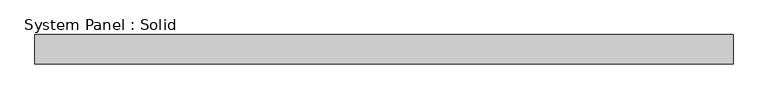
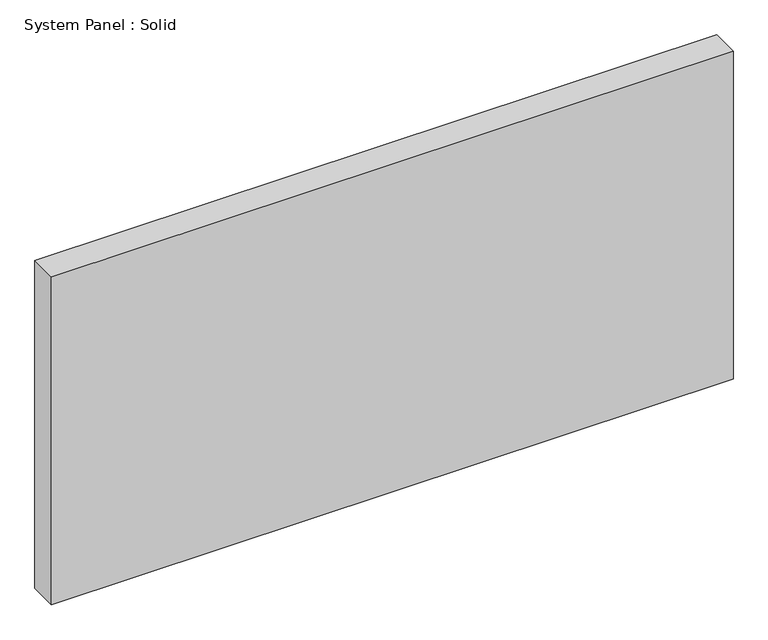
"""IFC4 building model written with IfcOpenShell, lengths in millimetres: plate geometry, System Panel : Solid."""

from ifc_helpers import new_model, si_unit, origin, origin_with_axes, place, context, project, spatial, polyline, outline, extrude, source, transform, mapped, element, save


def system_panel_solid_1c6a8c02(model_context):
    return source(origin(), model_context, "Body", "SweptSolid", [
        extrude(outline(polyline([(712.5000001, -10.5), (-712.5000001, -10.5), (-712.5000001, 49.5), (712.5000001, 49.5), (712.5000001, -10.5)])), origin_with_axes(), (0.0, 0.0, 1.0), 725.0),
    ])


if __name__ == "__main__":
    model = new_model("IFC4")
    model_context = context("Model", 3, world=origin())
    ifc_project = project(units=[si_unit("LENGTHUNIT", "METRE", prefix="MILLI")], contexts=[model_context])
    site = spatial("IfcSite", under=ifc_project)
    building = spatial("IfcBuilding", under=site)
    placement = place(None, origin())
    system_panel_solid_shape = system_panel_solid_1c6a8c02(model_context)
    element("IfcPlate", 1, ObjectType="System Panel : Solid", at=placement, inside=building, context=model_context, shape_type="MappedRepresentation", body=[
        mapped(system_panel_solid_shape, transform((0.0, 0.0, 0.0), x_axis=(1.0, 0.0, 0.0), y_axis=(0.0, 1.0, 0.0), z_axis=(0.0, 0.0, 1.0))),
    ])
    save(model, "model.ifc")

# Revit data of these elements
# Project information
#   Project Issue Date = "Issue Date"
#   Project Status = "Project Status"
#   Client Name = "Owner"
#   Project Address = "Enter address here"
#   Project Name = "Project Name"
#   Project Number = "Project Number"
# Type "System Panel : Solid"
#   Keynote = "H11"
#   Construction Type Id = "MDOOR"
#   Analytic Construction = "Metal"
#   Visual Light Transmittance = 0
#   Solar Heat Gain Coefficient = 0
#   Heat Transfer Coefficient (U) = 3.7021 W/(m²·K)
# Element 1 (IfcPlate, "System Panel : Solid")
#   Materials on its faces: "Default"
# Materials
#   "Default": class "Miscellaneous", colour RGB 127 127 127, transparency 0, Comments = "Rendering appearance not upgraded ", Cost = 0
